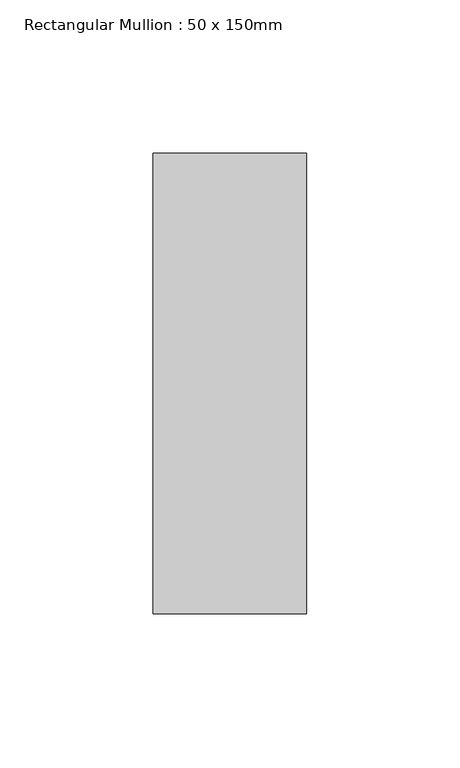
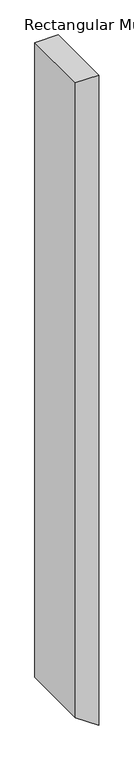
"""IFC4 building model written with IfcOpenShell, lengths in millimetres: member geometry, Rectangular Mullion : 50 x 150mm."""

import ifcopenshell
import ifcopenshell.guid

model = None  # the IFC model being written
_history = None  # IfcOwnerHistory: only IFC2X3 demands one
_inside = {}  # id of a spatial element -> (the spatial element, [elements in it])
_under = {}  # id of a project, library or spatial element -> (it, [spatial elements below it])
_declared = {}  # id of a project -> (the project, [libraries it declares])
_typed = {}  # id of a type object -> (the type object, [elements of that type])
_made_of = {}  # id of a material, layer set ... -> (it, [elements and type objects made of it])


def new_model(schema):
    """Start an empty IFC model of exactly this schema.

    Asked for "IFC4X3", IfcOpenShell would pick the latest addendum, in which some entities
    have other attributes; the version numbers below select the first issue.
    IFC2X3 requires an IfcOwnerHistory on every rooted entity: one is made here for all.
    """
    global model, _history
    if schema == "IFC4X3":
        model = ifcopenshell.file(schema_version=(4, 3, 0, 0))
    else:
        model = ifcopenshell.file(schema=schema)
    _inside.clear()
    _under.clear()
    _declared.clear()
    _typed.clear()
    _made_of.clear()
    _history = None
    if model.schema == "IFC2X3":
        org = make("IfcOrganization", Name="unknown")
        user = make(
            "IfcPersonAndOrganization",
            ThePerson=make("IfcPerson", FamilyName="unknown"),
            TheOrganization=org,
        )
        app = make(
            "IfcApplication",
            ApplicationDeveloper=org,
            Version="unknown",
            ApplicationFullName="unknown",
            ApplicationIdentifier="unknown",
        )
        _history = make(
            "IfcOwnerHistory",
            OwningUser=user,
            OwningApplication=app,
            ChangeAction="ADDED",
            CreationDate=0,
        )
    return model


def make(cls, **values):
    """One entity of the class cls with the attributes given. An attribute that is None is left unset."""
    return model.create_entity(
        cls, **{name: value for name, value in values.items() if value is not None}
    )


def rooted(cls, **values):
    """An entity with a GlobalId (a new one), such as an element, a storey or a relation."""
    return make(cls, GlobalId=ifcopenshell.guid.new(), OwnerHistory=_history, **values)


def si_unit(unit_type, name, prefix=None):
    """IfcSIUnit, for example si_unit("LENGTHUNIT", "METRE", prefix="MILLI")."""
    return make("IfcSIUnit", UnitType=unit_type, Prefix=prefix, Name=name)


def assignment(units):
    """IfcUnitAssignment: the units of a project."""
    return None if units is None else make("IfcUnitAssignment", Units=units)


def point(xyz):
    """IfcCartesianPoint."""
    return None if xyz is None else make("IfcCartesianPoint", Coordinates=xyz)


def direction(xyz):
    """IfcDirection."""
    return None if xyz is None else make("IfcDirection", DirectionRatios=xyz)


def frame(location, z_axis=None, x_axis=None):
    """IfcAxis2Placement3D, a coordinate frame: its origin and axes. An axis left out is left unset."""
    return make(
        "IfcAxis2Placement3D",
        Location=point(location),
        Axis=direction(z_axis),
        RefDirection=direction(x_axis),
    )


def origin():
    """The frame at (0, 0, 0) with its axes left unset."""
    return frame((0.0, 0.0, 0.0))


def place(relative_to, where):
    """IfcLocalPlacement: puts the frame where relative to a parent placement (None: the world)."""
    return make(
        "IfcLocalPlacement", PlacementRelTo=relative_to, RelativePlacement=where
    )


def context(
    kind, dimensions, precision=None, world=None, true_north=None, identifier=None
):
    """IfcGeometricRepresentationContext, for example the 3D "Model" context."""
    return make(
        "IfcGeometricRepresentationContext",
        ContextIdentifier=identifier,
        ContextType=kind,
        CoordinateSpaceDimension=dimensions,
        Precision=precision,
        WorldCoordinateSystem=world,
        TrueNorth=true_north,
    )


def project(units=None, contexts=None):
    """IfcProject with its units and contexts."""
    return rooted(
        "IfcProject",
        Name="project",
        RepresentationContexts=contexts,
        UnitsInContext=assignment(units),
    )


def spatial(cls, under=None, at=None, **own):
    """A site, building, storey or space (cls), placed at a placement, below another one or the project."""
    s = rooted(cls, ObjectPlacement=at, **own)
    if under is not None:
        _under.setdefault(under.id(), (under, []))[1].append(s)
    return s


def polyline(points):
    """IfcPolyline through the points."""
    return make("IfcPolyline", Points=[point(p) for p in points])


def outline(outer, holes=None, kind="AREA"):
    """IfcArbitraryClosedProfileDef: a profile drawn as a closed curve; with holes, ...WithVoids."""
    if holes is None:
        return make("IfcArbitraryClosedProfileDef", ProfileType=kind, OuterCurve=outer)
    return make(
        "IfcArbitraryProfileDefWithVoids",
        ProfileType=kind,
        OuterCurve=outer,
        InnerCurves=holes,
    )


def extrude(swept, where, along, depth):
    """IfcExtrudedAreaSolid: the profile swept, set in the frame where, extruded along a direction by depth."""
    return make(
        "IfcExtrudedAreaSolid",
        SweptArea=swept,
        Position=where,
        ExtrudedDirection=direction(along),
        Depth=depth,
    )


def shape(context_of_items, identifier, shape_type, items):
    """IfcShapeRepresentation: the items that make up one representation, for example the "Body"."""
    return make(
        "IfcShapeRepresentation",
        ContextOfItems=context_of_items,
        RepresentationIdentifier=identifier,
        RepresentationType=shape_type,
        Items=items,
    )


def source(mapping_origin, context_of_items, identifier, shape_type, items):
    """IfcRepresentationMap: a shape defined once, which mapped items show again and again."""
    return make(
        "IfcRepresentationMap",
        MappingOrigin=mapping_origin,
        MappedRepresentation=shape(context_of_items, identifier, shape_type, items),
    )


def transform(
    local_origin,
    x_axis=None,
    y_axis=None,
    z_axis=None,
    scale=None,
    scale2=None,
    scale3=None,
    uniform=True,
):
    """IfcCartesianTransformationOperator3D, or its non-uniform kind. x_axis, y_axis, z_axis: its Axis1, 2, 3."""
    if uniform:
        return make(
            "IfcCartesianTransformationOperator3D",
            Axis1=direction(x_axis),
            Axis2=direction(y_axis),
            LocalOrigin=point(local_origin),
            Scale=scale,
            Axis3=direction(z_axis),
        )
    return make(
        "IfcCartesianTransformationOperator3DnonUniform",
        Axis1=direction(x_axis),
        Axis2=direction(y_axis),
        LocalOrigin=point(local_origin),
        Scale=scale,
        Axis3=direction(z_axis),
        Scale2=scale2,
        Scale3=scale3,
    )


def mapped(mapping_source, mapping_target):
    """IfcMappedItem: shows the shape of a source again, moved by a transform."""
    return make(
        "IfcMappedItem", MappingSource=mapping_source, MappingTarget=mapping_target
    )


def made_of(thing, what):
    """Note that an element or type object is made of a material, layer set ...; save() writes the relation."""
    if what is not None:
        _made_of.setdefault(what.id(), (what, []))[1].append(thing)
    return thing


def element(
    cls,
    number,
    at=None,
    inside=None,
    cuts=None,
    type_object=None,
    material=None,
    context=None,
    identifier="Body",
    shape_type=None,
    held_by="IfcProductDefinitionShape",
    body=None,
    shapes=None,
    **own,
):
    """One element of the class cls, such as IfcWall. Its Tag is "e" and its number.

    at: its placement. inside: the storey or other place that contains it. cuts: it is an
    opening in that element (IfcRelVoidsElement). A single representation is given by context,
    identifier, shape_type and body (its items); several are given by shapes. held_by: the class
    of the entity that holds the representations. save() writes the other relations.
    """
    e = rooted(cls, Tag="e%d" % number, ObjectPlacement=at, **own)
    if body is not None:
        shapes = [shape(context, identifier, shape_type, body)]
    if shapes is not None:
        e.Representation = make(held_by, Representations=shapes)
    if inside is not None:
        _inside.setdefault(inside.id(), (inside, []))[1].append(e)
    if cuts is not None:
        rooted(
            "IfcRelVoidsElement", RelatingBuildingElement=cuts, RelatedOpeningElement=e
        )
    if type_object is not None:
        _typed.setdefault(type_object.id(), (type_object, []))[1].append(e)
    return made_of(e, material)


def aggregate(whole, parts):
    """IfcRelAggregates: a whole, such as a stair, and the parts it consists of."""
    return rooted("IfcRelAggregates", RelatingObject=whole, RelatedObjects=parts)


def save(model, path):
    """Write the relations noted so far, then the file.

    IfcRelAggregates (storeys below a building ...), IfcRelContainedInSpatialStructure (elements
    in a storey), IfcRelDefinesByType, IfcRelAssociatesMaterial and IfcRelDeclares: one each for
    every whole, place, type object, material and project.
    """
    for whole, parts in _under.values():
        aggregate(whole, parts)
    for where, things in _inside.values():
        rooted(
            "IfcRelContainedInSpatialStructure",
            RelatedElements=things,
            RelatingStructure=where,
        )
    for kind, things in _typed.values():
        rooted("IfcRelDefinesByType", RelatedObjects=things, RelatingType=kind)
    for what, things in _made_of.values():
        rooted("IfcRelAssociatesMaterial", RelatedObjects=things, RelatingMaterial=what)
    for by, libraries in _declared.values():
        rooted("IfcRelDeclares", RelatingContext=by, RelatedDefinitions=libraries)
    model.write(path)


def rectangular_mullion_50_x_150mm_93a95515(model_context):
    return source(origin(), model_context, "Body", "SweptSolid", [
        extrude(outline(polyline([(0.0, 25.0), (0.0, -25.0), (-1431.7258818, -25.0), (-1466.7362587, 25.0), (0.0, 25.0)])), frame((0.0, -75.0, 0.0), z_axis=(0.0, 1.0, 0.0), x_axis=(0.0, 0.0, 1.0)), (0.0, 0.0, 1.0), 150.0),
    ])


if __name__ == "__main__":
    model = new_model("IFC4")
    model_context = context("Model", 3, world=origin())
    ifc_project = project(units=[si_unit("LENGTHUNIT", "METRE", prefix="MILLI")], contexts=[model_context])
    site = spatial("IfcSite", under=ifc_project)
    building = spatial("IfcBuilding", under=site)
    placement = place(None, origin())
    rectangular_mullion_50_x_150mm_shape = rectangular_mullion_50_x_150mm_93a95515(model_context)
    element("IfcMember", 1, ObjectType="Rectangular Mullion : 50 x 150mm", at=placement, inside=building, context=model_context, shape_type="MappedRepresentation", body=[
        mapped(rectangular_mullion_50_x_150mm_shape, transform((0.0, 0.0, 0.0), x_axis=(1.0, 0.0, 0.0), y_axis=(0.0, 1.0, 0.0), z_axis=(0.0, 0.0, 1.0))),
    ])
    save(model, "model.ifc")

# Revit data of these elements
# Type "Rectangular Mullion : 50 x 150mm"
#   built-in parameter 1007304 = 0.492126 (stored number, unit not read)
#   built-in parameter 1007301 = 0.082021 (stored number, unit not read)
#   built-in parameter 1007300 = 0.082021 (stored number, unit not read)
# Element 1 (IfcMember, "Rectangular Mullion : 50 x 150mm")
#   Materials on its faces: "Aluminium"
# Materials
#   "Aluminium": class "Metal", colour RGB 247 247 247, transparency 0, Description = "Aluminium 6061", Cost = 0
